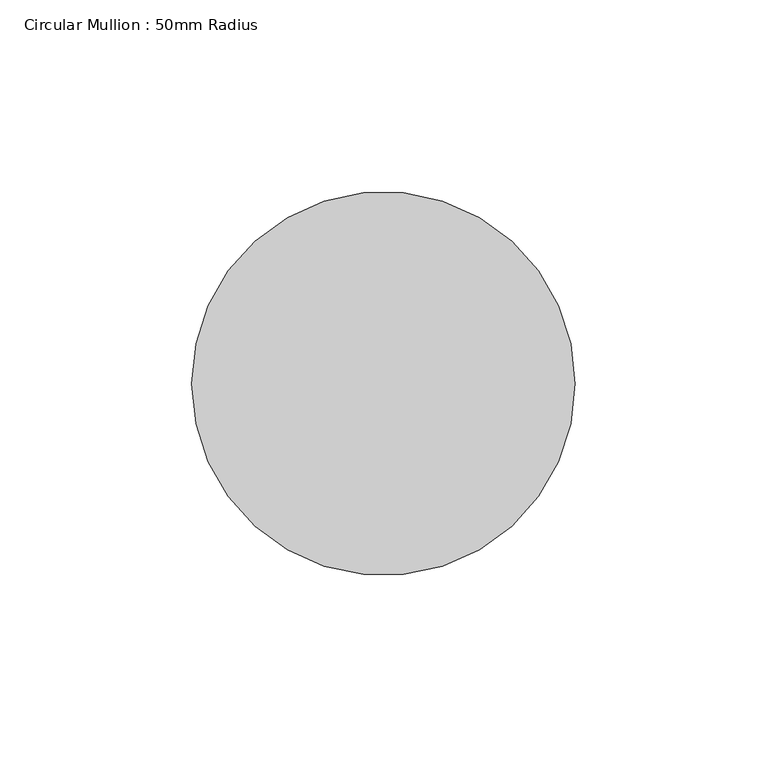
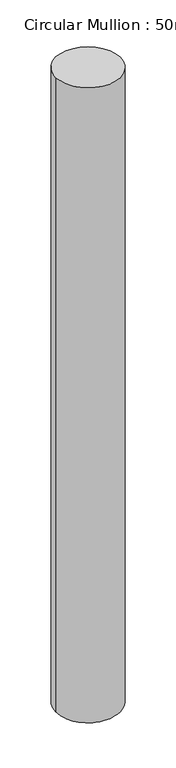
"""IFC4 building model written with IfcOpenShell, lengths in millimetres: member geometry, Circular Mullion : 50mm Radius."""

import ifcopenshell
import ifcopenshell.guid

model = None  # the IFC model being written
_history = None  # IfcOwnerHistory: only IFC2X3 demands one
_inside = {}  # id of a spatial element -> (the spatial element, [elements in it])
_under = {}  # id of a project, library or spatial element -> (it, [spatial elements below it])
_declared = {}  # id of a project -> (the project, [libraries it declares])
_typed = {}  # id of a type object -> (the type object, [elements of that type])
_made_of = {}  # id of a material, layer set ... -> (it, [elements and type objects made of it])


def new_model(schema):
    """Start an empty IFC model of exactly this schema.

    Asked for "IFC4X3", IfcOpenShell would pick the latest addendum, in which some entities
    have other attributes; the version numbers below select the first issue.
    IFC2X3 requires an IfcOwnerHistory on every rooted entity: one is made here for all.
    """
    global model, _history
    if schema == "IFC4X3":
        model = ifcopenshell.file(schema_version=(4, 3, 0, 0))
    else:
        model = ifcopenshell.file(schema=schema)
    _inside.clear()
    _under.clear()
    _declared.clear()
    _typed.clear()
    _made_of.clear()
    _history = None
    if model.schema == "IFC2X3":
        org = make("IfcOrganization", Name="unknown")
        user = make(
            "IfcPersonAndOrganization",
            ThePerson=make("IfcPerson", FamilyName="unknown"),
            TheOrganization=org,
        )
        app = make(
            "IfcApplication",
            ApplicationDeveloper=org,
            Version="unknown",
            ApplicationFullName="unknown",
            ApplicationIdentifier="unknown",
        )
        _history = make(
            "IfcOwnerHistory",
            OwningUser=user,
            OwningApplication=app,
            ChangeAction="ADDED",
            CreationDate=0,
        )
    return model


def make(cls, **values):
    """One entity of the class cls with the attributes given. An attribute that is None is left unset."""
    return model.create_entity(
        cls, **{name: value for name, value in values.items() if value is not None}
    )


def rooted(cls, **values):
    """An entity with a GlobalId (a new one), such as an element, a storey or a relation."""
    return make(cls, GlobalId=ifcopenshell.guid.new(), OwnerHistory=_history, **values)


def si_unit(unit_type, name, prefix=None):
    """IfcSIUnit, for example si_unit("LENGTHUNIT", "METRE", prefix="MILLI")."""
    return make("IfcSIUnit", UnitType=unit_type, Prefix=prefix, Name=name)


def assignment(units):
    """IfcUnitAssignment: the units of a project."""
    return None if units is None else make("IfcUnitAssignment", Units=units)


def point(xyz):
    """IfcCartesianPoint."""
    return None if xyz is None else make("IfcCartesianPoint", Coordinates=xyz)


def direction(xyz):
    """IfcDirection."""
    return None if xyz is None else make("IfcDirection", DirectionRatios=xyz)


def frame(location, z_axis=None, x_axis=None):
    """IfcAxis2Placement3D, a coordinate frame: its origin and axes. An axis left out is left unset."""
    return make(
        "IfcAxis2Placement3D",
        Location=point(location),
        Axis=direction(z_axis),
        RefDirection=direction(x_axis),
    )


def origin():
    """The frame at (0, 0, 0) with its axes left unset."""
    return frame((0.0, 0.0, 0.0))


def place(relative_to, where):
    """IfcLocalPlacement: puts the frame where relative to a parent placement (None: the world)."""
    return make(
        "IfcLocalPlacement", PlacementRelTo=relative_to, RelativePlacement=where
    )


def context(
    kind, dimensions, precision=None, world=None, true_north=None, identifier=None
):
    """IfcGeometricRepresentationContext, for example the 3D "Model" context."""
    return make(
        "IfcGeometricRepresentationContext",
        ContextIdentifier=identifier,
        ContextType=kind,
        CoordinateSpaceDimension=dimensions,
        Precision=precision,
        WorldCoordinateSystem=world,
        TrueNorth=true_north,
    )


def project(units=None, contexts=None):
    """IfcProject with its units and contexts."""
    return rooted(
        "IfcProject",
        Name="project",
        RepresentationContexts=contexts,
        UnitsInContext=assignment(units),
    )


def spatial(cls, under=None, at=None, **own):
    """A site, building, storey or space (cls), placed at a placement, below another one or the project."""
    s = rooted(cls, ObjectPlacement=at, **own)
    if under is not None:
        _under.setdefault(under.id(), (under, []))[1].append(s)
    return s


def ellipse_curve(where, semi_axis1, semi_axis2):
    """IfcEllipse in the frame where."""
    return make(
        "IfcEllipse", Position=where, SemiAxis1=semi_axis1, SemiAxis2=semi_axis2
    )


def shape(context_of_items, identifier, shape_type, items):
    """IfcShapeRepresentation: the items that make up one representation, for example the "Body"."""
    return make(
        "IfcShapeRepresentation",
        ContextOfItems=context_of_items,
        RepresentationIdentifier=identifier,
        RepresentationType=shape_type,
        Items=items,
    )


def source(mapping_origin, context_of_items, identifier, shape_type, items):
    """IfcRepresentationMap: a shape defined once, which mapped items show again and again."""
    return make(
        "IfcRepresentationMap",
        MappingOrigin=mapping_origin,
        MappedRepresentation=shape(context_of_items, identifier, shape_type, items),
    )


def transform(
    local_origin,
    x_axis=None,
    y_axis=None,
    z_axis=None,
    scale=None,
    scale2=None,
    scale3=None,
    uniform=True,
):
    """IfcCartesianTransformationOperator3D, or its non-uniform kind. x_axis, y_axis, z_axis: its Axis1, 2, 3."""
    if uniform:
        return make(
            "IfcCartesianTransformationOperator3D",
            Axis1=direction(x_axis),
            Axis2=direction(y_axis),
            LocalOrigin=point(local_origin),
            Scale=scale,
            Axis3=direction(z_axis),
        )
    return make(
        "IfcCartesianTransformationOperator3DnonUniform",
        Axis1=direction(x_axis),
        Axis2=direction(y_axis),
        LocalOrigin=point(local_origin),
        Scale=scale,
        Axis3=direction(z_axis),
        Scale2=scale2,
        Scale3=scale3,
    )


def mapped(mapping_source, mapping_target):
    """IfcMappedItem: shows the shape of a source again, moved by a transform."""
    return make(
        "IfcMappedItem", MappingSource=mapping_source, MappingTarget=mapping_target
    )


def made_of(thing, what):
    """Note that an element or type object is made of a material, layer set ...; save() writes the relation."""
    if what is not None:
        _made_of.setdefault(what.id(), (what, []))[1].append(thing)
    return thing


def element(
    cls,
    number,
    at=None,
    inside=None,
    cuts=None,
    type_object=None,
    material=None,
    context=None,
    identifier="Body",
    shape_type=None,
    held_by="IfcProductDefinitionShape",
    body=None,
    shapes=None,
    **own,
):
    """One element of the class cls, such as IfcWall. Its Tag is "e" and its number.

    at: its placement. inside: the storey or other place that contains it. cuts: it is an
    opening in that element (IfcRelVoidsElement). A single representation is given by context,
    identifier, shape_type and body (its items); several are given by shapes. held_by: the class
    of the entity that holds the representations. save() writes the other relations.
    """
    e = rooted(cls, Tag="e%d" % number, ObjectPlacement=at, **own)
    if body is not None:
        shapes = [shape(context, identifier, shape_type, body)]
    if shapes is not None:
        e.Representation = make(held_by, Representations=shapes)
    if inside is not None:
        _inside.setdefault(inside.id(), (inside, []))[1].append(e)
    if cuts is not None:
        rooted(
            "IfcRelVoidsElement", RelatingBuildingElement=cuts, RelatedOpeningElement=e
        )
    if type_object is not None:
        _typed.setdefault(type_object.id(), (type_object, []))[1].append(e)
    return made_of(e, material)


def aggregate(whole, parts):
    """IfcRelAggregates: a whole, such as a stair, and the parts it consists of."""
    return rooted("IfcRelAggregates", RelatingObject=whole, RelatedObjects=parts)


def save(model, path):
    """Write the relations noted so far, then the file.

    IfcRelAggregates (storeys below a building ...), IfcRelContainedInSpatialStructure (elements
    in a storey), IfcRelDefinesByType, IfcRelAssociatesMaterial and IfcRelDeclares: one each for
    every whole, place, type object, material and project.
    """
    for whole, parts in _under.values():
        aggregate(whole, parts)
    for where, things in _inside.values():
        rooted(
            "IfcRelContainedInSpatialStructure",
            RelatedElements=things,
            RelatingStructure=where,
        )
    for kind, things in _typed.values():
        rooted("IfcRelDefinesByType", RelatedObjects=things, RelatingType=kind)
    for what, things in _made_of.values():
        rooted("IfcRelAssociatesMaterial", RelatedObjects=things, RelatingMaterial=what)
    for by, libraries in _declared.values():
        rooted("IfcRelDeclares", RelatingContext=by, RelatedDefinitions=libraries)
    model.write(path)


def plane_surface(at):
    """IfcPlane: the flat surface through the origin of the frame at, square to its z axis."""
    return make("IfcPlane", Position=at)


def cylinder_surface(at, radius):
    """IfcCylindricalSurface: all points at the distance radius from the z axis of the frame at."""
    return make("IfcCylindricalSurface", Position=at, Radius=radius)


def advanced_brep(points, edges, surfaces, faces):
    """IfcAdvancedBrep: a solid bounded by faces that lie on surfaces and meet in shared edges.

    An edge is (start, end): straight between two places in points (the first is 0);
    or (start, end, curve); or (start, end, curve, False) where it runs against its curve.
    A face is (place in surfaces, loops), or (place, loops, False) where it looks against
    its surface's normal. A loop lists edges by number (the first is 1), with a minus sign
    where the edge is run from its end to its start. The first loop is the outer one.
    """
    corners = [point(p) for p in points]
    vertices = [make("IfcVertexPoint", VertexGeometry=c) for c in corners]
    made = []
    for start, end, *more in edges:
        made.append(
            make(
                "IfcEdgeCurve",
                EdgeStart=vertices[start],
                EdgeEnd=vertices[end],
                EdgeGeometry=more[0] if more else make("IfcPolyline", Points=[corners[start], corners[end]]),
                SameSense=more[1] if len(more) > 1 else True,
            )
        )
    hull = []
    for where, loops, *sense in faces:
        bounds = []
        for j, loop in enumerate(loops):
            ring = [make("IfcOrientedEdge", EdgeElement=made[abs(k) - 1], Orientation=k > 0) for k in loop]
            bounds.append(
                make(
                    "IfcFaceOuterBound" if j == 0 else "IfcFaceBound",
                    Bound=make("IfcEdgeLoop", EdgeList=ring),
                    Orientation=True,
                )
            )
        hull.append(make("IfcAdvancedFace", Bounds=bounds, FaceSurface=surfaces[where], SameSense=sense[0] if sense else True))
    return make("IfcAdvancedBrep", Outer=make("IfcClosedShell", CfsFaces=hull))


def circular_mullion_50mm_radius_744fddef(model_context):
    return source(origin(), model_context, "Body", "AdvancedBrep", [
        advanced_brep(
        [(-100.0, 0.0, 1.8482168), (0.0, 0.0, 0.0), (0.0, 0.0, -1034.7815152), (-100.0, 0.0, -1036.6930999)],
        [
            (0, 1, ellipse_curve(frame((-50.0, 0.0, 0.9241084), z_axis=(-0.018474423292371336, -0.022283849408849206, -0.9995809750788267), x_axis=(-0.6379688106381792, -0.769517980551751, 0.028946057770653698)), 50.02096, 50.0)),
            (1, 2),
            (2, 3, ellipse_curve(frame((-50.0, 0.0, -1035.7373075), z_axis=(-0.01910727919818019, -0.023047200203584826, 0.99955176876659), x_axis=(0.637950170111081, 0.7694954963478744, 0.029937627754738606)), 50.0224216, 50.0)),
            (3, 0),
            (1, 0, ellipse_curve(frame((-50.0, 0.0, 0.9241084), z_axis=(-0.018474423292371336, -0.022283849408849206, -0.9995809750788267), x_axis=(-0.6379688106381792, -0.769517980551751, 0.028946057770653698)), 50.02096, 50.0)),
            (3, 2, ellipse_curve(frame((-50.0, 0.0, -1035.7373075), z_axis=(-0.01910727919818019, -0.023047200203584826, 0.99955176876659), x_axis=(0.637950170111081, 0.7694954963478744, 0.029937627754738606)), 50.0224216, 50.0)),
        ],
        [
            cylinder_surface(frame((-50.0, 0.0, 0.0), z_axis=(0.0, 0.0, 1.0), x_axis=(1.0, 0.0, 0.0)), 50.0),
            plane_surface(frame((-234.6474036, 194.5344082, 0.0), z_axis=(0.018474423292371336, 0.022283849408849206, 0.9995809750788267), x_axis=(0.6379688106381795, 0.7695179805517508, -0.02894605777065301))),
            plane_surface(frame((-234.6474036, 194.5344082, -1034.7815152), z_axis=(0.019107279198180192, 0.02304720020358483, -0.9995517687665902), x_axis=(0.6379501701110809, 0.7694954963478745, 0.029937627754739186))),
        ],
        [
            (0, [[1, 2, 3, 4]]),
            (0, [[5, -4, 6, -2]]),
            (1, [[-1, -5]]),
            (2, [[-6, -3]]),
        ],
    ),
    ])


if __name__ == "__main__":
    model = new_model("IFC4")
    model_context = context("Model", 3, world=origin())
    ifc_project = project(units=[si_unit("LENGTHUNIT", "METRE", prefix="MILLI")], contexts=[model_context])
    site = spatial("IfcSite", under=ifc_project)
    building = spatial("IfcBuilding", under=site)
    placement = place(None, origin())
    circular_mullion_50mm_radius_shape = circular_mullion_50mm_radius_744fddef(model_context)
    element("IfcMember", 1, ObjectType="Circular Mullion : 50mm Radius", at=placement, inside=building, context=model_context, shape_type="MappedRepresentation", body=[
        mapped(circular_mullion_50mm_radius_shape, transform((0.0, 0.0, 0.0), x_axis=(1.0, 0.0, 0.0), y_axis=(0.0, 1.0, 0.0), z_axis=(0.0, 0.0, 1.0))),
    ])
    save(model, "model.ifc")

# Revit data of these elements
# Type "Circular Mullion : 50mm Radius"
#   built-in parameter 1007350 = 0.164042 (stored number, unit not read)
# Element 1 (IfcMember, "Circular Mullion : 50mm Radius")
#   Materials on its faces: "Aluminium"
# Materials
#   "Aluminium": class "Metal", colour RGB 247 247 247, transparency 0, Description = "Aluminium 6061", Cost = 0
